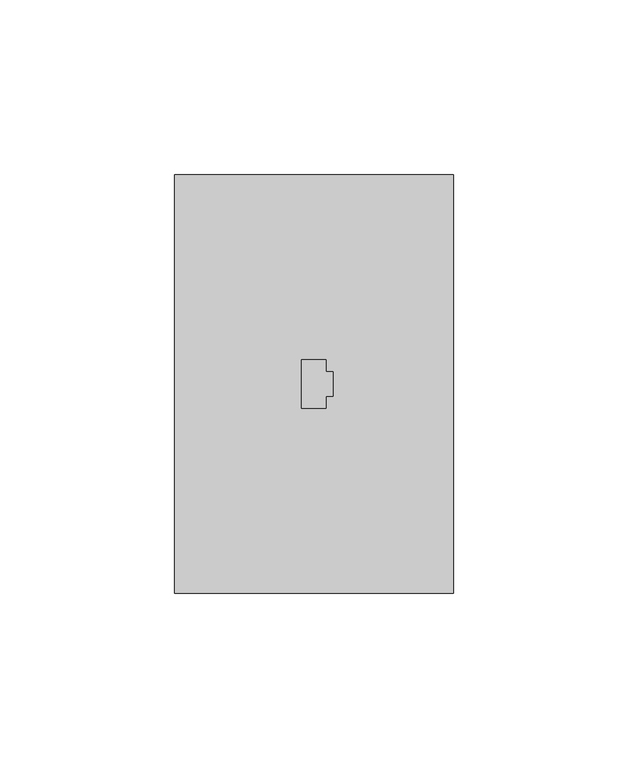
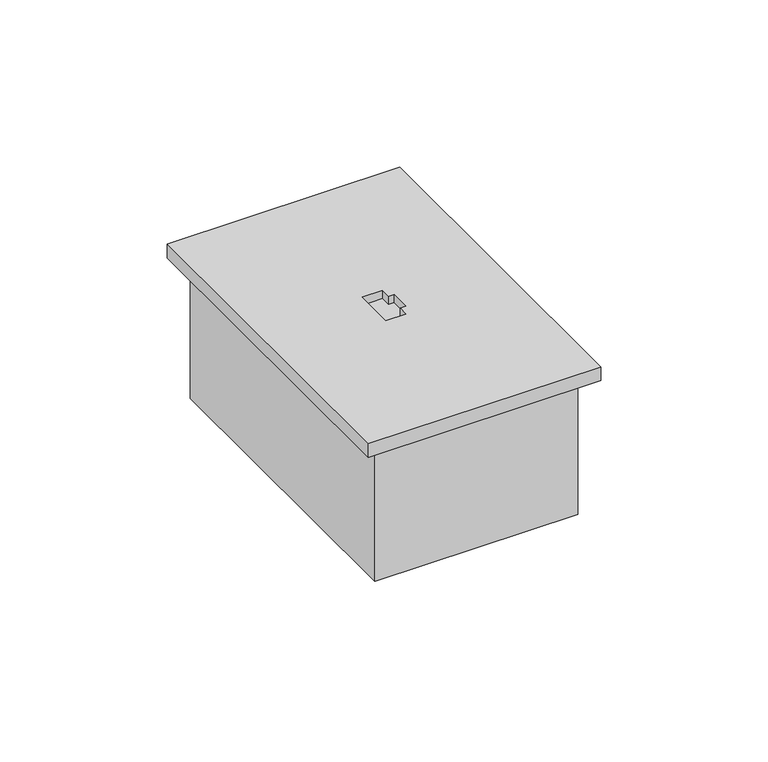
"""IFC4 building model written with IfcOpenShell, lengths in millimetres: proxy geometry, CAIXA VERTICE V7 : Rede."""

from ifc_helpers import new_model, si_unit, origin, place, context, project, spatial, faceted_brep, source, transform, mapped, element, save


def electrical_fixtures_76e978e4(model_context):
    return source(origin(), model_context, "Body", "Brep", [
        faceted_brep([(33.0, -1047.0, -48.0), (-33.0, -1047.0, -48.0), (-33.0, -1153.0, -48.0), (33.0, -1153.0, -48.0), (35.0, -1155.0, -50.0), (-35.0, -1155.0, -50.0), (-35.0, -1045.0, -50.0), (35.0, -1045.0, -50.0), (35.0, -1155.0, 0.0), (-35.0, -1155.0, 0.0), (-35.0, -1045.0, 0.0), (35.0, -1045.0, 0.0), (33.0, -1153.0, 0.0), (-33.0, -1153.0, 0.0), (-33.0, -1047.0, 0.0), (33.0, -1047.0, 0.0)], [[[0, 1, 2, 3]], [[4, 5, 6, 7]], [[4, 8, 9, 5]], [[9, 10, 6, 5]], [[10, 11, 7, 6]], [[11, 8, 4, 7]], [[8, 11, 10, 9], [12, 13, 14, 15]], [[15, 0, 3, 12]], [[14, 1, 0, 15]], [[13, 2, 1, 14]], [[12, 3, 2, 13]]]),
        faceted_brep([(40.0, -1160.0, 5.0), (40.0, -1040.0, 5.0), (-40.0, -1040.0, 5.0), (-40.0, -1160.0, 5.0), (5.5, -1103.5, 5.0), (3.5, -1103.5, 5.0), (3.5, -1107.0, 5.0), (-3.5, -1107.0, 5.0), (-3.5, -1093.0, 5.0), (3.5, -1093.0, 5.0), (3.5, -1096.5, 5.0), (5.5, -1096.5, 5.0), (-40.0, -1160.0, 0.0), (-40.0, -1040.0, 0.0), (40.0, -1040.0, 0.0), (40.0, -1160.0, 0.0), (5.5, -1103.5, 2.0), (5.5, -1096.5, 2.0), (3.5, -1103.5, 2.0), (3.5, -1107.0, 2.0), (3.5, -1096.5, 2.0), (3.5, -1093.0, 2.0), (-3.5, -1093.0, 2.0), (-3.5, -1107.0, 2.0)], [[[0, 1, 2, 3], [4, 5, 6, 7, 8, 9, 10, 11]], [[12, 13, 14, 15]], [[3, 12, 15, 0]], [[2, 13, 12, 3]], [[1, 14, 13, 2]], [[0, 15, 14, 1]], [[16, 4, 11, 17]], [[18, 5, 4, 16]], [[19, 6, 5, 18]], [[19, 18, 16, 17, 20, 21, 22, 23]], [[23, 7, 6, 19]], [[22, 8, 7, 23]], [[21, 9, 8, 22]], [[20, 10, 9, 21]], [[17, 11, 10, 20]]]),
    ])


if __name__ == "__main__":
    model = new_model("IFC4")
    model_context = context("Model", 3, world=origin())
    ifc_project = project(units=[si_unit("LENGTHUNIT", "METRE", prefix="MILLI")], contexts=[model_context])
    site = spatial("IfcSite", under=ifc_project)
    building = spatial("IfcBuilding", under=site)
    placement = place(None, origin())
    electrical_fixtures_shape = electrical_fixtures_76e978e4(model_context)
    element("IfcBuildingElementProxy", 1, Name="CAIXA VERTICE V7 : Rede", ObjectType="CAIXA VERTICE V7 : Rede", at=placement, inside=building, context=model_context, shape_type="MappedRepresentation", body=[
        mapped(electrical_fixtures_shape, transform((0.0, 0.0, 0.0), x_axis=(1.0, 0.0, 0.0), y_axis=(0.0, 1.0, 0.0), z_axis=(0.0, 0.0, 1.0))),
    ])
    save(model, "model.ifc")

# Revit data of these elements
# Type "CAIXA VERTICE V7 : Rede"
#   URL = "www.facebook.com/verticetreinamentos"
#   SEÇÃO [instance default] = ""
#   Rotação [instance default] = 0.00°
#   LARGURA DA TAMPA = 0.08 m
#   BORDA = 0.01 m
#   ALTURA DE INSTALAÇÃO [instance default] = 1.10 m
#   Distância Anotação [instance default] = 0.0015 m
#   ALTURA DA TAMPA = 0.12 m
#   Vertical [instance default] = yes
#   VER SEÇÃO [instance default] = no
#   SHADE ESQ [instance default] = no
#   SHADE DIR [instance default] = yes
#   HORIZONTAL [instance default] = no
#   ANDAR COM A LEGENDA [instance default] = 0
#   Material Tampa [instance default] = Plástico, branco opaco
#   Caixa = element 1798521
#   Anotação = element 1798536
#   Default Elevation = 0
# Element 1 (IfcBuildingElementProxy, "CAIXA VERTICE V7 : Rede")
#   SEÇÃO = "2"
#   VER SEÇÃO = yes
#   Materials on its faces: "Plástico, branco opaco"
# Materials
#   "Plástico, branco opaco": class "Plástico", colour RGB 120 120 120, transparency 0, Description = "Plastic, generic, opaque white", Cost = 0
